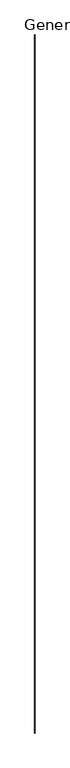
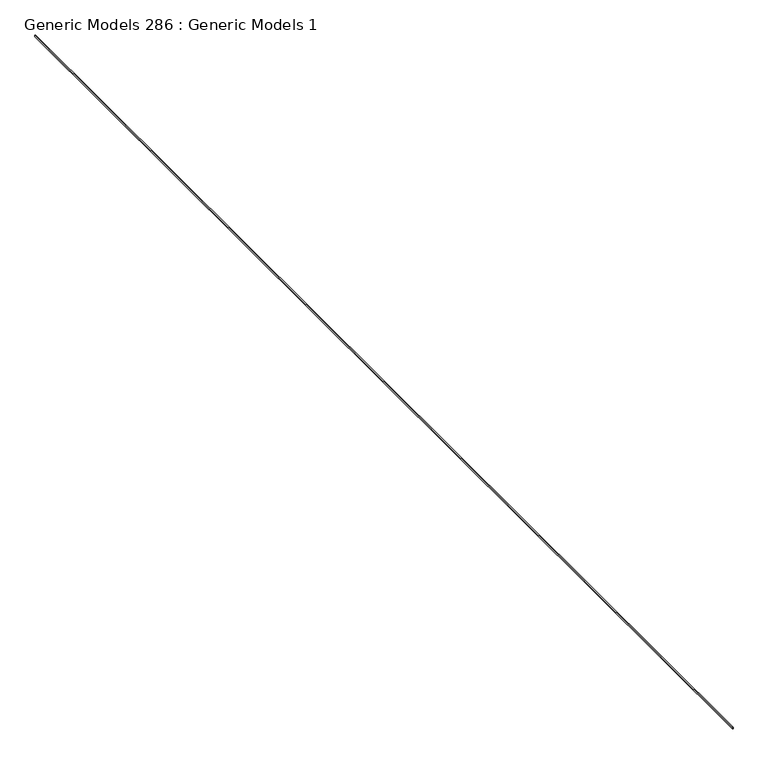
"""IFC4 building model written with IfcOpenShell, lengths in millimetres: proxy geometry, Generic Models 286 : Generic Models 1."""

import ifcopenshell
import ifcopenshell.guid

model = None  # the IFC model being written
_history = None  # IfcOwnerHistory: only IFC2X3 demands one
_inside = {}  # id of a spatial element -> (the spatial element, [elements in it])
_under = {}  # id of a project, library or spatial element -> (it, [spatial elements below it])
_declared = {}  # id of a project -> (the project, [libraries it declares])
_typed = {}  # id of a type object -> (the type object, [elements of that type])
_made_of = {}  # id of a material, layer set ... -> (it, [elements and type objects made of it])


def new_model(schema):
    """Start an empty IFC model of exactly this schema.

    Asked for "IFC4X3", IfcOpenShell would pick the latest addendum, in which some entities
    have other attributes; the version numbers below select the first issue.
    IFC2X3 requires an IfcOwnerHistory on every rooted entity: one is made here for all.
    """
    global model, _history
    if schema == "IFC4X3":
        model = ifcopenshell.file(schema_version=(4, 3, 0, 0))
    else:
        model = ifcopenshell.file(schema=schema)
    _inside.clear()
    _under.clear()
    _declared.clear()
    _typed.clear()
    _made_of.clear()
    _history = None
    if model.schema == "IFC2X3":
        org = make("IfcOrganization", Name="unknown")
        user = make(
            "IfcPersonAndOrganization",
            ThePerson=make("IfcPerson", FamilyName="unknown"),
            TheOrganization=org,
        )
        app = make(
            "IfcApplication",
            ApplicationDeveloper=org,
            Version="unknown",
            ApplicationFullName="unknown",
            ApplicationIdentifier="unknown",
        )
        _history = make(
            "IfcOwnerHistory",
            OwningUser=user,
            OwningApplication=app,
            ChangeAction="ADDED",
            CreationDate=0,
        )
    return model


def make(cls, **values):
    """One entity of the class cls with the attributes given. An attribute that is None is left unset."""
    return model.create_entity(
        cls, **{name: value for name, value in values.items() if value is not None}
    )


def rooted(cls, **values):
    """An entity with a GlobalId (a new one), such as an element, a storey or a relation."""
    return make(cls, GlobalId=ifcopenshell.guid.new(), OwnerHistory=_history, **values)


def si_unit(unit_type, name, prefix=None):
    """IfcSIUnit, for example si_unit("LENGTHUNIT", "METRE", prefix="MILLI")."""
    return make("IfcSIUnit", UnitType=unit_type, Prefix=prefix, Name=name)


def assignment(units):
    """IfcUnitAssignment: the units of a project."""
    return None if units is None else make("IfcUnitAssignment", Units=units)


def point(xyz):
    """IfcCartesianPoint."""
    return None if xyz is None else make("IfcCartesianPoint", Coordinates=xyz)


def direction(xyz):
    """IfcDirection."""
    return None if xyz is None else make("IfcDirection", DirectionRatios=xyz)


def frame(location, z_axis=None, x_axis=None):
    """IfcAxis2Placement3D, a coordinate frame: its origin and axes. An axis left out is left unset."""
    return make(
        "IfcAxis2Placement3D",
        Location=point(location),
        Axis=direction(z_axis),
        RefDirection=direction(x_axis),
    )


def frame_2d(location, x_axis=None):
    """IfcAxis2Placement2D, a coordinate frame in the plane: its origin and x axis."""
    return make(
        "IfcAxis2Placement2D", Location=point(location), RefDirection=direction(x_axis)
    )


def origin():
    """The frame at (0, 0, 0) with its axes left unset."""
    return frame((0.0, 0.0, 0.0))


def place(relative_to, where):
    """IfcLocalPlacement: puts the frame where relative to a parent placement (None: the world)."""
    return make(
        "IfcLocalPlacement", PlacementRelTo=relative_to, RelativePlacement=where
    )


def context(
    kind, dimensions, precision=None, world=None, true_north=None, identifier=None
):
    """IfcGeometricRepresentationContext, for example the 3D "Model" context."""
    return make(
        "IfcGeometricRepresentationContext",
        ContextIdentifier=identifier,
        ContextType=kind,
        CoordinateSpaceDimension=dimensions,
        Precision=precision,
        WorldCoordinateSystem=world,
        TrueNorth=true_north,
    )


def project(units=None, contexts=None):
    """IfcProject with its units and contexts."""
    return rooted(
        "IfcProject",
        Name="project",
        RepresentationContexts=contexts,
        UnitsInContext=assignment(units),
    )


def spatial(cls, under=None, at=None, **own):
    """A site, building, storey or space (cls), placed at a placement, below another one or the project."""
    s = rooted(cls, ObjectPlacement=at, **own)
    if under is not None:
        _under.setdefault(under.id(), (under, []))[1].append(s)
    return s


def polyline(points):
    """IfcPolyline through the points."""
    return make("IfcPolyline", Points=[point(p) for p in points])


def circle_curve(where, radius):
    """IfcCircle in the frame where."""
    return make("IfcCircle", Position=where, Radius=radius)


def trimmed(basis, trim1, trim2, sense, master):
    """IfcTrimmedCurve: the piece of a basis curve between two trims."""
    return make(
        "IfcTrimmedCurve",
        BasisCurve=basis,
        Trim1=trim1,
        Trim2=trim2,
        SenseAgreement=sense,
        MasterRepresentation=master,
    )


def segment(curve, same_sense, transition):
    """IfcCompositeCurveSegment."""
    return make(
        "IfcCompositeCurveSegment",
        Transition=transition,
        SameSense=same_sense,
        ParentCurve=curve,
    )


def composite_curve(segments, self_intersect=None):
    """IfcCompositeCurve: segments joined end to end."""
    return make("IfcCompositeCurve", Segments=segments, SelfIntersect=self_intersect)


def outline(outer, holes=None, kind="AREA"):
    """IfcArbitraryClosedProfileDef: a profile drawn as a closed curve; with holes, ...WithVoids."""
    if holes is None:
        return make("IfcArbitraryClosedProfileDef", ProfileType=kind, OuterCurve=outer)
    return make(
        "IfcArbitraryProfileDefWithVoids",
        ProfileType=kind,
        OuterCurve=outer,
        InnerCurves=holes,
    )


def extrude(swept, where, along, depth):
    """IfcExtrudedAreaSolid: the profile swept, set in the frame where, extruded along a direction by depth."""
    return make(
        "IfcExtrudedAreaSolid",
        SweptArea=swept,
        Position=where,
        ExtrudedDirection=direction(along),
        Depth=depth,
    )


def shape(context_of_items, identifier, shape_type, items):
    """IfcShapeRepresentation: the items that make up one representation, for example the "Body"."""
    return make(
        "IfcShapeRepresentation",
        ContextOfItems=context_of_items,
        RepresentationIdentifier=identifier,
        RepresentationType=shape_type,
        Items=items,
    )


def source(mapping_origin, context_of_items, identifier, shape_type, items):
    """IfcRepresentationMap: a shape defined once, which mapped items show again and again."""
    return make(
        "IfcRepresentationMap",
        MappingOrigin=mapping_origin,
        MappedRepresentation=shape(context_of_items, identifier, shape_type, items),
    )


def transform(
    local_origin,
    x_axis=None,
    y_axis=None,
    z_axis=None,
    scale=None,
    scale2=None,
    scale3=None,
    uniform=True,
):
    """IfcCartesianTransformationOperator3D, or its non-uniform kind. x_axis, y_axis, z_axis: its Axis1, 2, 3."""
    if uniform:
        return make(
            "IfcCartesianTransformationOperator3D",
            Axis1=direction(x_axis),
            Axis2=direction(y_axis),
            LocalOrigin=point(local_origin),
            Scale=scale,
            Axis3=direction(z_axis),
        )
    return make(
        "IfcCartesianTransformationOperator3DnonUniform",
        Axis1=direction(x_axis),
        Axis2=direction(y_axis),
        LocalOrigin=point(local_origin),
        Scale=scale,
        Axis3=direction(z_axis),
        Scale2=scale2,
        Scale3=scale3,
    )


def mapped(mapping_source, mapping_target):
    """IfcMappedItem: shows the shape of a source again, moved by a transform."""
    return make(
        "IfcMappedItem", MappingSource=mapping_source, MappingTarget=mapping_target
    )


def made_of(thing, what):
    """Note that an element or type object is made of a material, layer set ...; save() writes the relation."""
    if what is not None:
        _made_of.setdefault(what.id(), (what, []))[1].append(thing)
    return thing


def element(
    cls,
    number,
    at=None,
    inside=None,
    cuts=None,
    type_object=None,
    material=None,
    context=None,
    identifier="Body",
    shape_type=None,
    held_by="IfcProductDefinitionShape",
    body=None,
    shapes=None,
    **own,
):
    """One element of the class cls, such as IfcWall. Its Tag is "e" and its number.

    at: its placement. inside: the storey or other place that contains it. cuts: it is an
    opening in that element (IfcRelVoidsElement). A single representation is given by context,
    identifier, shape_type and body (its items); several are given by shapes. held_by: the class
    of the entity that holds the representations. save() writes the other relations.
    """
    e = rooted(cls, Tag="e%d" % number, ObjectPlacement=at, **own)
    if body is not None:
        shapes = [shape(context, identifier, shape_type, body)]
    if shapes is not None:
        e.Representation = make(held_by, Representations=shapes)
    if inside is not None:
        _inside.setdefault(inside.id(), (inside, []))[1].append(e)
    if cuts is not None:
        rooted(
            "IfcRelVoidsElement", RelatingBuildingElement=cuts, RelatedOpeningElement=e
        )
    if type_object is not None:
        _typed.setdefault(type_object.id(), (type_object, []))[1].append(e)
    return made_of(e, material)


def aggregate(whole, parts):
    """IfcRelAggregates: a whole, such as a stair, and the parts it consists of."""
    return rooted("IfcRelAggregates", RelatingObject=whole, RelatedObjects=parts)


def save(model, path):
    """Write the relations noted so far, then the file.

    IfcRelAggregates (storeys below a building ...), IfcRelContainedInSpatialStructure (elements
    in a storey), IfcRelDefinesByType, IfcRelAssociatesMaterial and IfcRelDeclares: one each for
    every whole, place, type object, material and project.
    """
    for whole, parts in _under.values():
        aggregate(whole, parts)
    for where, things in _inside.values():
        rooted(
            "IfcRelContainedInSpatialStructure",
            RelatedElements=things,
            RelatingStructure=where,
        )
    for kind, things in _typed.values():
        rooted("IfcRelDefinesByType", RelatedObjects=things, RelatingType=kind)
    for what, things in _made_of.values():
        rooted("IfcRelAssociatesMaterial", RelatedObjects=things, RelatingMaterial=what)
    for by, libraries in _declared.values():
        rooted("IfcRelDeclares", RelatingContext=by, RelatedDefinitions=libraries)
    model.write(path)


def generic_models_286_generic_models_1_937c068a(model_context):
    return source(origin(), model_context, "Body", "SweptSolid", [
        extrude(outline(composite_curve([segment(polyline([(129485.9589141, 1443.4012224), (129476.4339141, 1443.4012224)]), True, "CONTINUOUS"), segment(trimmed(circle_curve(frame_2d((129473.5191736, 1446.5762224)), 4.3100275), [point((129476.4339141, 1443.4012224))], [point((129476.4339141, 1449.7512224))], True, "CARTESIAN"), True, "CONTINUOUS"), segment(polyline([(129476.4339141, 1449.7512224), (129485.9589141, 1449.7512224)]), True, "CONTINUOUS"), segment(trimmed(circle_curve(frame_2d((129483.0441736, 1446.5762224)), 4.3100275), [point((129485.9589141, 1449.7512224))], [point((129485.9589141, 1443.4012224))], False, "CARTESIAN"), True, "CONTINUOUS")], self_intersect=False)), frame((0.0, 306.6963299, 0.0), z_axis=(0.0, 1.0, 0.0), x_axis=(0.0, 0.0, 1.0)), (0.0, 0.0, 1.0), 7886.7),
    ])


if __name__ == "__main__":
    model = new_model("IFC4")
    model_context = context("Model", 3, world=origin())
    ifc_project = project(units=[si_unit("LENGTHUNIT", "METRE", prefix="MILLI")], contexts=[model_context])
    site = spatial("IfcSite", under=ifc_project)
    building = spatial("IfcBuilding", under=site)
    placement = place(None, origin())
    generic_models_286_generic_models_1_shape = generic_models_286_generic_models_1_937c068a(model_context)
    element("IfcBuildingElementProxy", 1, Name="Generic Models 286 : Generic Models 1", ObjectType="Generic Models 286 : Generic Models 1", at=placement, inside=building, context=model_context, shape_type="MappedRepresentation", body=[
        mapped(generic_models_286_generic_models_1_shape, transform((0.0, 0.0, 0.0), x_axis=(1.0, 0.0, 0.0), y_axis=(0.0, 1.0, 0.0), z_axis=(0.0, 0.0, 1.0))),
    ])
    save(model, "model.ifc")

# Revit data of these elements
# Element 1 (IfcBuildingElementProxy, "Generic Models 286 : Generic Models 1")
#   Materials on its faces: "_SEALANT JOINT"
# Materials
#   "_SEALANT JOINT": class "Generic", colour RGB 190 220 196, transparency 0, Cost = 0
